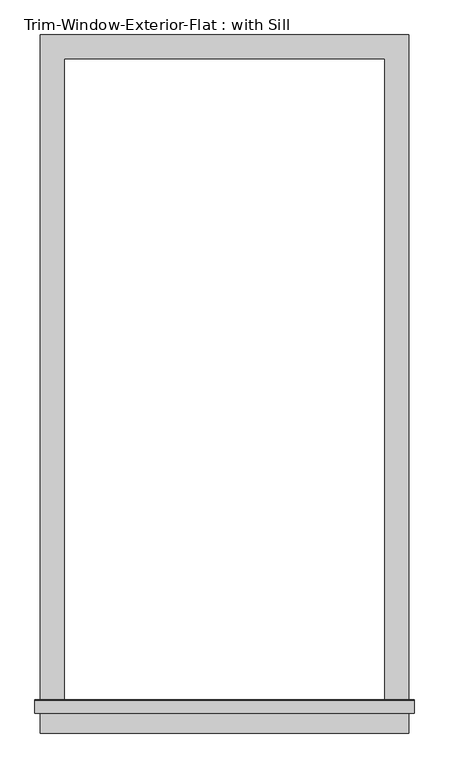
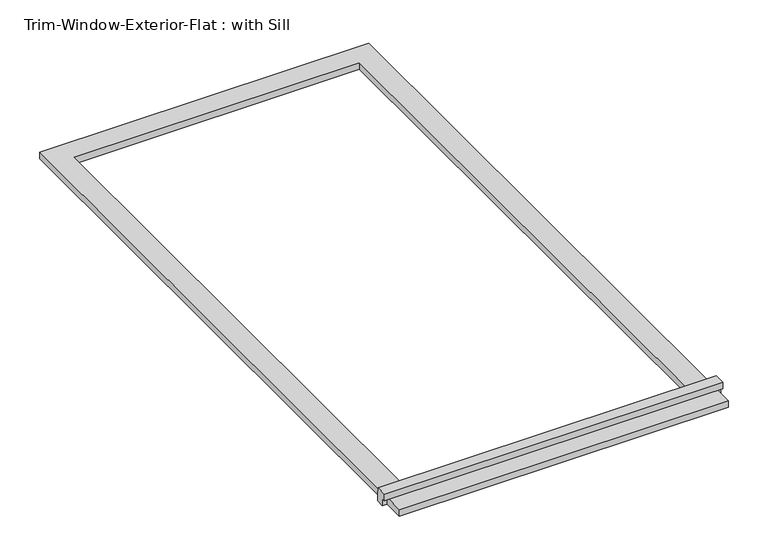
"""IFC4 building model written with IfcOpenShell, lengths in millimetres: proxy geometry, Trim-Window-Exterior-Flat : with Sill."""

from ifc_helpers import new_model, si_unit, frame, origin, origin_with_axes, place, context, project, spatial, polyline, outline, extrude, source, transform, mapped, element, save


def trim_window_exterior_flat_with_sill_42432628(model_context):
    return source(origin(), model_context, "Body", "SweptSolid", [
        extrude(outline(polyline([(438.15, -1546.1823709), (438.15, -1603.3323709), (-438.15, -1603.3323709), (-438.15, -1546.1823709), (438.15, -1546.1823709)])), origin_with_axes(), (0.0, 0.0, 1.0), 19.05),
        extrude(outline(polyline([(-1555.75, 38.1), (-1526.4580645, 38.1), (-1524.0, 19.05), (-1524.0, 0.0), (-1546.1823709, 0.0), (-1546.1823709, 19.05), (-1555.75, 19.05), (-1555.75, 38.1)])), frame((-450.85, 0.0, 0.0), z_axis=(1.0, 0.0, 0.0), x_axis=(0.0, 1.0, 0.0)), (0.0, 0.0, 1.0), 901.7),
        extrude(outline(polyline([(-438.15, 57.15), (438.15, 57.15), (438.15, -1524.0), (381.0, -1524.0), (381.0, 0.0), (-381.0, 0.0), (-381.0, -1524.0), (-438.15, -1524.0), (-438.15, 57.15)])), origin_with_axes(), (0.0, 0.0, 1.0), 19.05),
    ])


if __name__ == "__main__":
    model = new_model("IFC4")
    model_context = context("Model", 3, world=origin())
    ifc_project = project(units=[si_unit("LENGTHUNIT", "METRE", prefix="MILLI")], contexts=[model_context])
    site = spatial("IfcSite", under=ifc_project)
    building = spatial("IfcBuilding", under=site)
    placement = place(None, origin())
    trim_window_exterior_flat_with_sill_shape = trim_window_exterior_flat_with_sill_42432628(model_context)
    element("IfcBuildingElementProxy", 1, Name="Trim-Window-Exterior-Flat : with Sill", ObjectType="Trim-Window-Exterior-Flat : with Sill", at=placement, inside=building, context=model_context, shape_type="MappedRepresentation", body=[
        mapped(trim_window_exterior_flat_with_sill_shape, transform((0.0, 0.0, 0.0), x_axis=(1.0, 0.0, 0.0), y_axis=(0.0, 1.0, 0.0), z_axis=(0.0, 0.0, 1.0))),
    ])
    save(model, "model.ifc")

# Revit data of these elements
# Type "Trim-Window-Exterior-Flat : with Sill"
#   Trim Width = 0' - 2 1/4"
#   Trim Thickness_Picture Frame = 0' - 1 1/4"
#   Trim Thickness_with Sill = 0' - 0 3/4"
#   Sill Thickness = 0' - 1 1/4"
#   Opening Width [instance default] = 2' - 0"
#   Opening Height [instance default] = 3' - 0"
#   Default Elevation = 4' - 0"
#   Sill = yes
#   Picture Frame = no
#   Trim Material [instance default] = none
# Element 1 (IfcBuildingElementProxy, "Trim-Window-Exterior-Flat : with Sill")
#   Opening Width = 2' - 6"
#   Opening Height = 5' - 0"
#   Trim Material = Clad - White
#   Materials on its faces: "Clad - White"
# Materials
#   "Clad - White": class "Wood", colour RGB 242 242 238, transparency 0, Cost = 0
